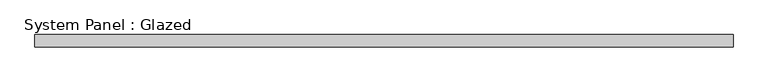
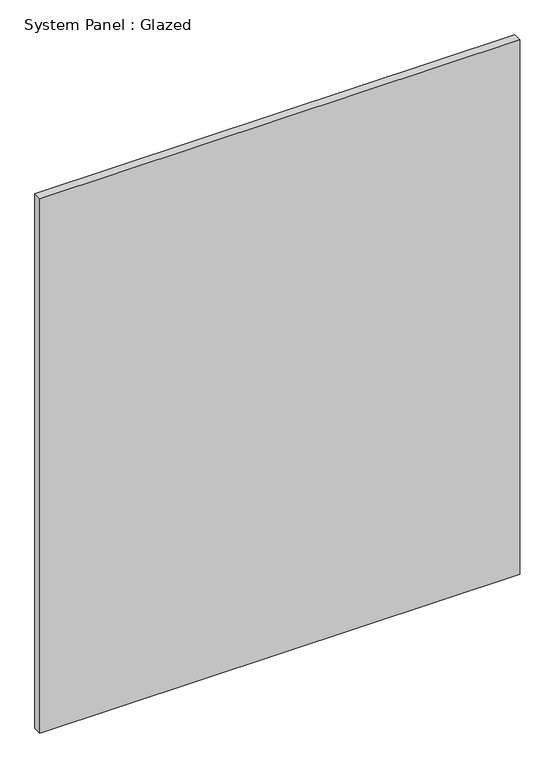
"""IFC4 building model written with IfcOpenShell, lengths in millimetres: plate geometry, System Panel : Glazed."""

import ifcopenshell
import ifcopenshell.guid

model = None  # the IFC model being written
_history = None  # IfcOwnerHistory: only IFC2X3 demands one
_inside = {}  # id of a spatial element -> (the spatial element, [elements in it])
_under = {}  # id of a project, library or spatial element -> (it, [spatial elements below it])
_declared = {}  # id of a project -> (the project, [libraries it declares])
_typed = {}  # id of a type object -> (the type object, [elements of that type])
_made_of = {}  # id of a material, layer set ... -> (it, [elements and type objects made of it])


def new_model(schema):
    """Start an empty IFC model of exactly this schema.

    Asked for "IFC4X3", IfcOpenShell would pick the latest addendum, in which some entities
    have other attributes; the version numbers below select the first issue.
    IFC2X3 requires an IfcOwnerHistory on every rooted entity: one is made here for all.
    """
    global model, _history
    if schema == "IFC4X3":
        model = ifcopenshell.file(schema_version=(4, 3, 0, 0))
    else:
        model = ifcopenshell.file(schema=schema)
    _inside.clear()
    _under.clear()
    _declared.clear()
    _typed.clear()
    _made_of.clear()
    _history = None
    if model.schema == "IFC2X3":
        org = make("IfcOrganization", Name="unknown")
        user = make(
            "IfcPersonAndOrganization",
            ThePerson=make("IfcPerson", FamilyName="unknown"),
            TheOrganization=org,
        )
        app = make(
            "IfcApplication",
            ApplicationDeveloper=org,
            Version="unknown",
            ApplicationFullName="unknown",
            ApplicationIdentifier="unknown",
        )
        _history = make(
            "IfcOwnerHistory",
            OwningUser=user,
            OwningApplication=app,
            ChangeAction="ADDED",
            CreationDate=0,
        )
    return model


def make(cls, **values):
    """One entity of the class cls with the attributes given. An attribute that is None is left unset."""
    return model.create_entity(
        cls, **{name: value for name, value in values.items() if value is not None}
    )


def rooted(cls, **values):
    """An entity with a GlobalId (a new one), such as an element, a storey or a relation."""
    return make(cls, GlobalId=ifcopenshell.guid.new(), OwnerHistory=_history, **values)


def si_unit(unit_type, name, prefix=None):
    """IfcSIUnit, for example si_unit("LENGTHUNIT", "METRE", prefix="MILLI")."""
    return make("IfcSIUnit", UnitType=unit_type, Prefix=prefix, Name=name)


def assignment(units):
    """IfcUnitAssignment: the units of a project."""
    return None if units is None else make("IfcUnitAssignment", Units=units)


def point(xyz):
    """IfcCartesianPoint."""
    return None if xyz is None else make("IfcCartesianPoint", Coordinates=xyz)


def direction(xyz):
    """IfcDirection."""
    return None if xyz is None else make("IfcDirection", DirectionRatios=xyz)


def frame(location, z_axis=None, x_axis=None):
    """IfcAxis2Placement3D, a coordinate frame: its origin and axes. An axis left out is left unset."""
    return make(
        "IfcAxis2Placement3D",
        Location=point(location),
        Axis=direction(z_axis),
        RefDirection=direction(x_axis),
    )


def origin():
    """The frame at (0, 0, 0) with its axes left unset."""
    return frame((0.0, 0.0, 0.0))


def origin_with_axes():
    """The frame at (0, 0, 0) with the z axis (0, 0, 1) and the x axis (1, 0, 0) written out."""
    return frame((0.0, 0.0, 0.0), z_axis=(0.0, 0.0, 1.0), x_axis=(1.0, 0.0, 0.0))


def place(relative_to, where):
    """IfcLocalPlacement: puts the frame where relative to a parent placement (None: the world)."""
    return make(
        "IfcLocalPlacement", PlacementRelTo=relative_to, RelativePlacement=where
    )


def context(
    kind, dimensions, precision=None, world=None, true_north=None, identifier=None
):
    """IfcGeometricRepresentationContext, for example the 3D "Model" context."""
    return make(
        "IfcGeometricRepresentationContext",
        ContextIdentifier=identifier,
        ContextType=kind,
        CoordinateSpaceDimension=dimensions,
        Precision=precision,
        WorldCoordinateSystem=world,
        TrueNorth=true_north,
    )


def project(units=None, contexts=None):
    """IfcProject with its units and contexts."""
    return rooted(
        "IfcProject",
        Name="project",
        RepresentationContexts=contexts,
        UnitsInContext=assignment(units),
    )


def spatial(cls, under=None, at=None, **own):
    """A site, building, storey or space (cls), placed at a placement, below another one or the project."""
    s = rooted(cls, ObjectPlacement=at, **own)
    if under is not None:
        _under.setdefault(under.id(), (under, []))[1].append(s)
    return s


def polyline(points):
    """IfcPolyline through the points."""
    return make("IfcPolyline", Points=[point(p) for p in points])


def outline(outer, holes=None, kind="AREA"):
    """IfcArbitraryClosedProfileDef: a profile drawn as a closed curve; with holes, ...WithVoids."""
    if holes is None:
        return make("IfcArbitraryClosedProfileDef", ProfileType=kind, OuterCurve=outer)
    return make(
        "IfcArbitraryProfileDefWithVoids",
        ProfileType=kind,
        OuterCurve=outer,
        InnerCurves=holes,
    )


def extrude(swept, where, along, depth):
    """IfcExtrudedAreaSolid: the profile swept, set in the frame where, extruded along a direction by depth."""
    return make(
        "IfcExtrudedAreaSolid",
        SweptArea=swept,
        Position=where,
        ExtrudedDirection=direction(along),
        Depth=depth,
    )


def shape(context_of_items, identifier, shape_type, items):
    """IfcShapeRepresentation: the items that make up one representation, for example the "Body"."""
    return make(
        "IfcShapeRepresentation",
        ContextOfItems=context_of_items,
        RepresentationIdentifier=identifier,
        RepresentationType=shape_type,
        Items=items,
    )


def source(mapping_origin, context_of_items, identifier, shape_type, items):
    """IfcRepresentationMap: a shape defined once, which mapped items show again and again."""
    return make(
        "IfcRepresentationMap",
        MappingOrigin=mapping_origin,
        MappedRepresentation=shape(context_of_items, identifier, shape_type, items),
    )


def transform(
    local_origin,
    x_axis=None,
    y_axis=None,
    z_axis=None,
    scale=None,
    scale2=None,
    scale3=None,
    uniform=True,
):
    """IfcCartesianTransformationOperator3D, or its non-uniform kind. x_axis, y_axis, z_axis: its Axis1, 2, 3."""
    if uniform:
        return make(
            "IfcCartesianTransformationOperator3D",
            Axis1=direction(x_axis),
            Axis2=direction(y_axis),
            LocalOrigin=point(local_origin),
            Scale=scale,
            Axis3=direction(z_axis),
        )
    return make(
        "IfcCartesianTransformationOperator3DnonUniform",
        Axis1=direction(x_axis),
        Axis2=direction(y_axis),
        LocalOrigin=point(local_origin),
        Scale=scale,
        Axis3=direction(z_axis),
        Scale2=scale2,
        Scale3=scale3,
    )


def mapped(mapping_source, mapping_target):
    """IfcMappedItem: shows the shape of a source again, moved by a transform."""
    return make(
        "IfcMappedItem", MappingSource=mapping_source, MappingTarget=mapping_target
    )


def made_of(thing, what):
    """Note that an element or type object is made of a material, layer set ...; save() writes the relation."""
    if what is not None:
        _made_of.setdefault(what.id(), (what, []))[1].append(thing)
    return thing


def element(
    cls,
    number,
    at=None,
    inside=None,
    cuts=None,
    type_object=None,
    material=None,
    context=None,
    identifier="Body",
    shape_type=None,
    held_by="IfcProductDefinitionShape",
    body=None,
    shapes=None,
    **own,
):
    """One element of the class cls, such as IfcWall. Its Tag is "e" and its number.

    at: its placement. inside: the storey or other place that contains it. cuts: it is an
    opening in that element (IfcRelVoidsElement). A single representation is given by context,
    identifier, shape_type and body (its items); several are given by shapes. held_by: the class
    of the entity that holds the representations. save() writes the other relations.
    """
    e = rooted(cls, Tag="e%d" % number, ObjectPlacement=at, **own)
    if body is not None:
        shapes = [shape(context, identifier, shape_type, body)]
    if shapes is not None:
        e.Representation = make(held_by, Representations=shapes)
    if inside is not None:
        _inside.setdefault(inside.id(), (inside, []))[1].append(e)
    if cuts is not None:
        rooted(
            "IfcRelVoidsElement", RelatingBuildingElement=cuts, RelatedOpeningElement=e
        )
    if type_object is not None:
        _typed.setdefault(type_object.id(), (type_object, []))[1].append(e)
    return made_of(e, material)


def aggregate(whole, parts):
    """IfcRelAggregates: a whole, such as a stair, and the parts it consists of."""
    return rooted("IfcRelAggregates", RelatingObject=whole, RelatedObjects=parts)


def save(model, path):
    """Write the relations noted so far, then the file.

    IfcRelAggregates (storeys below a building ...), IfcRelContainedInSpatialStructure (elements
    in a storey), IfcRelDefinesByType, IfcRelAssociatesMaterial and IfcRelDeclares: one each for
    every whole, place, type object, material and project.
    """
    for whole, parts in _under.values():
        aggregate(whole, parts)
    for where, things in _inside.values():
        rooted(
            "IfcRelContainedInSpatialStructure",
            RelatedElements=things,
            RelatingStructure=where,
        )
    for kind, things in _typed.values():
        rooted("IfcRelDefinesByType", RelatedObjects=things, RelatingType=kind)
    for what, things in _made_of.values():
        rooted("IfcRelAssociatesMaterial", RelatedObjects=things, RelatingMaterial=what)
    for by, libraries in _declared.values():
        rooted("IfcRelDeclares", RelatingContext=by, RelatedDefinitions=libraries)
    model.write(path)


def system_panel_glazed_3162bc82(model_context):
    return source(origin(), model_context, "Body", "SweptSolid", [
        extrude(outline(polyline([(718.0084626, 24.5), (-718.0084626, 24.5), (-718.0084626, 49.5), (718.0084626, 49.5), (718.0084626, 24.5)])), origin_with_axes(), (0.0, 0.0, 1.0), 1690.2939092),
    ])


if __name__ == "__main__":
    model = new_model("IFC4")
    model_context = context("Model", 3, world=origin())
    ifc_project = project(units=[si_unit("LENGTHUNIT", "METRE", prefix="MILLI")], contexts=[model_context])
    site = spatial("IfcSite", under=ifc_project)
    building = spatial("IfcBuilding", under=site)
    placement = place(None, origin())
    system_panel_glazed_shape = system_panel_glazed_3162bc82(model_context)
    element("IfcPlate", 1, ObjectType="System Panel : Glazed", at=placement, inside=building, context=model_context, shape_type="MappedRepresentation", body=[
        mapped(system_panel_glazed_shape, transform((0.0, 0.0, 0.0), x_axis=(1.0, 0.0, 0.0), y_axis=(0.0, 1.0, 0.0), z_axis=(0.0, 0.0, 1.0))),
    ])
    save(model, "model.ifc")

# Revit data of these elements
# Element 1 (IfcPlate, "System Panel : Glazed")
#   Materials on its faces: "Glass"
# Materials
#   "Glass": class "Glass", colour RGB 218 227 224, transparency 0.85, Description = "Soda Lime Glass", Cost = 0
